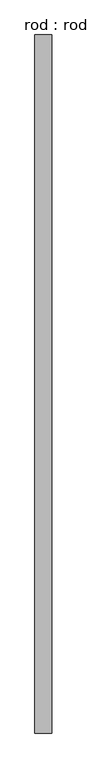
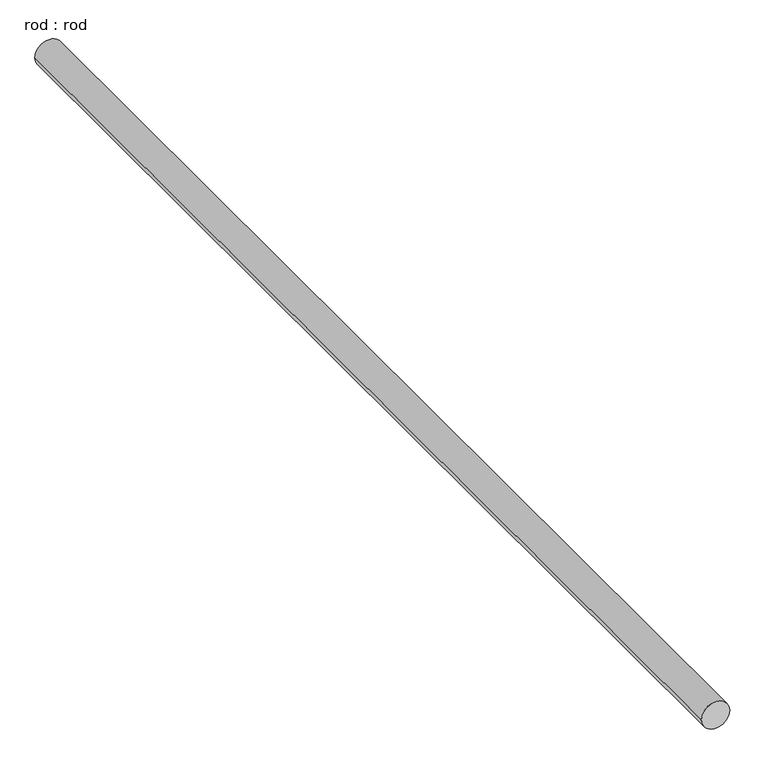
"""IFC4 building model written with IfcOpenShell, lengths in millimetres: proxy geometry, rod : rod."""

from ifc_helpers import new_model, si_unit, point, frame, frame_2d, origin, place, context, project, spatial, circle_curve, trimmed, segment, composite_curve, outline, extrude, source, transform, mapped, element, save


def rod_rod_7bf1a1de(model_context):
    return source(origin(), model_context, "Body", "SweptSolid", [
        extrude(outline(composite_curve([segment(trimmed(circle_curve(frame_2d((0.0108462, 0.0)), 200.0), [point((0.0108462, 200.0))], [point((0.0108462, -200.0))], False, "CARTESIAN"), True, "CONTINUOUS"), segment(trimmed(circle_curve(frame_2d((0.0108462, 0.0)), 200.0), [point((0.0108462, -200.0))], [point((0.0108462, 200.0))], False, "CARTESIAN"), True, "CONTINUOUS")], self_intersect=False)), frame((0.0, -4083.3496097, 0.0), z_axis=(0.0, 1.0, 0.0), x_axis=(0.0, 0.0, 1.0)), (0.0, 0.0, 1.0), 16352.1564501),
    ])


if __name__ == "__main__":
    model = new_model("IFC4")
    model_context = context("Model", 3, world=origin())
    ifc_project = project(units=[si_unit("LENGTHUNIT", "METRE", prefix="MILLI")], contexts=[model_context])
    site = spatial("IfcSite", under=ifc_project)
    building = spatial("IfcBuilding", under=site)
    placement = place(None, origin())
    rod_rod_shape = rod_rod_7bf1a1de(model_context)
    element("IfcBuildingElementProxy", 1, Name="rod : rod", ObjectType="rod : rod", at=placement, inside=building, context=model_context, shape_type="MappedRepresentation", body=[
        mapped(rod_rod_shape, transform((0.0, 0.0, 0.0), x_axis=(1.0, 0.0, 0.0), y_axis=(0.0, 1.0, 0.0), z_axis=(0.0, 0.0, 1.0))),
    ])
    save(model, "model.ifc")

# Revit data of these elements
# Type "rod : rod"
#   Default Elevation = 0
